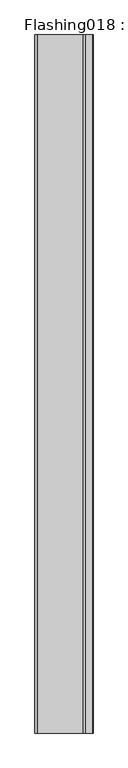
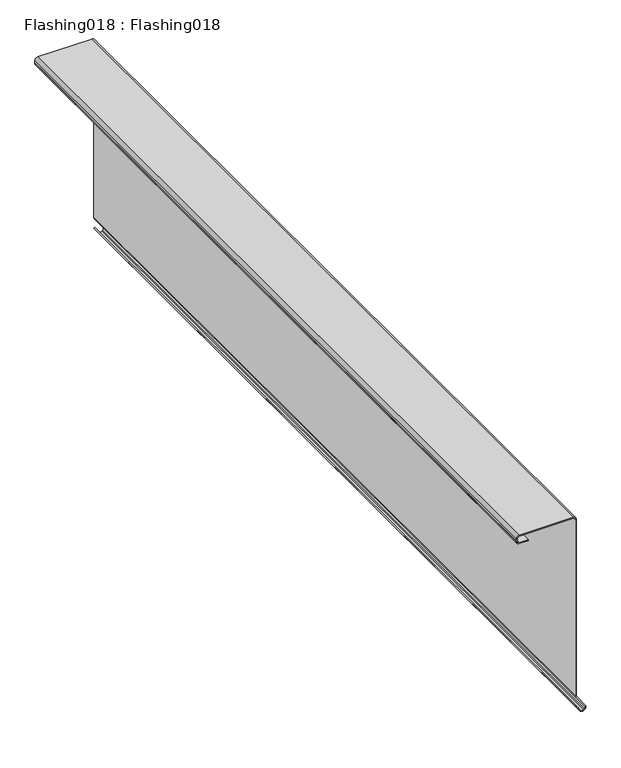
"""IFC4 building model written with IfcOpenShell, lengths in millimetres: proxy geometry, Flashing018 : Flashing018."""

from ifc_helpers import new_model, si_unit, point, frame, frame_2d, origin, place, context, project, spatial, polyline, circle_curve, trimmed, segment, composite_curve, outline, extrude, source, transform, mapped, element, save


def flashing018_flashing018_9543aaf0(model_context):
    return source(origin(), model_context, "Body", "SweptSolid", [
        extrude(outline(composite_curve([segment(polyline([(43036.8907248, 17759.2743151), (43051.477598, 17749.0170677), (43050.3271805, 17747.3810543), (43035.7403074, 17757.6383018)]), True, "CONTINUOUS"), segment(trimmed(circle_curve(frame_2d((43039.8127852, 17763.429789)), 7.08), [point((43035.7403074, 17757.6383018))], [point((43034.0825771, 17767.5880476))], False, "CARTESIAN"), True, "CONTINUOUS"), segment(polyline([(43034.0825771, 17767.5880476), (43035.3752562, 17769.3693991)]), True, "CONTINUOUS"), segment(trimmed(circle_curve(frame_2d((43041.1054643, 17765.2111405)), 7.08), [point((43035.3752562, 17769.3693991))], [point((43045.1570771, 17771.0172436))], False, "CARTESIAN"), True, "CONTINUOUS"), segment(polyline([(43045.1570771, 17771.0172436), (43075.4099277, 17749.9062098)]), True, "CONTINUOUS"), segment(trimmed(circle_curve(frame_2d((43077.1724938, 17752.4320286)), 3.08), [point((43075.4099277, 17749.9062098))], [point((43077.1724938, 17749.3520286))], True, "CARTESIAN"), True, "CONTINUOUS"), segment(polyline([(43077.1724938, 17749.3520286), (43524.4015043, 17749.3520286)]), True, "CONTINUOUS"), segment(trimmed(circle_curve(frame_2d((43524.4015043, 17742.2720286)), 7.08), [point((43524.4015043, 17749.3520286))], [point((43531.4815043, 17742.2720286))], False, "CARTESIAN"), True, "CONTINUOUS"), segment(polyline([(43531.4815043, 17742.2720286), (43531.4815043, 17612.9320286)]), True, "CONTINUOUS"), segment(trimmed(circle_curve(frame_2d((43524.4015043, 17612.9320286)), 7.08), [point((43531.4815043, 17612.9320286))], [point((43524.4015043, 17605.8520286))], False, "CARTESIAN"), True, "CONTINUOUS"), segment(polyline([(43524.4015043, 17605.8520286), (43517.995098, 17605.8520286)]), True, "CONTINUOUS"), segment(trimmed(circle_curve(frame_2d((43517.995098, 17612.9320286)), 7.08), [point((43517.995098, 17605.8520286))], [point((43510.915098, 17612.9320286))], False, "CARTESIAN"), True, "CONTINUOUS"), segment(polyline([(43510.915098, 17612.9320286), (43510.915098, 17634.2284935), (43512.915098, 17634.2284935), (43512.915098, 17612.9320286)]), True, "CONTINUOUS"), segment(trimmed(circle_curve(frame_2d((43517.995098, 17612.9320286)), 5.08), [point((43512.915098, 17612.9320286))], [point((43517.995098, 17607.8520286))], True, "CARTESIAN"), True, "CONTINUOUS"), segment(polyline([(43517.995098, 17607.8520286), (43524.4015043, 17607.8520286)]), True, "CONTINUOUS"), segment(trimmed(circle_curve(frame_2d((43524.4015043, 17612.9320286)), 5.08), [point((43524.4015043, 17607.8520286))], [point((43529.4815043, 17612.9320286))], True, "CARTESIAN"), True, "CONTINUOUS"), segment(polyline([(43529.4815043, 17612.9320286), (43529.4815043, 17742.2720286)]), True, "CONTINUOUS"), segment(trimmed(circle_curve(frame_2d((43524.4015043, 17742.2720286)), 5.08), [point((43529.4815043, 17742.2720286))], [point((43524.4015043, 17747.3520286))], True, "CARTESIAN"), True, "CONTINUOUS"), segment(polyline([(43524.4015043, 17747.3520286), (43077.1724938, 17747.3520286)]), True, "CONTINUOUS"), segment(trimmed(circle_curve(frame_2d((43077.1724938, 17752.4320286)), 5.08), [point((43077.1724938, 17747.3520286))], [point((43074.2654043, 17748.2660676))], False, "CARTESIAN"), True, "CONTINUOUS"), segment(polyline([(43074.2654043, 17748.2660676), (43044.0125537, 17769.3771014)]), True, "CONTINUOUS"), segment(trimmed(circle_curve(frame_2d((43041.1054643, 17765.2111405)), 5.08), [point((43044.0125537, 17769.3771014))], [point((43036.993959, 17768.1947498))], True, "CARTESIAN"), True, "CONTINUOUS"), segment(polyline([(43036.993959, 17768.1947498), (43035.7012799, 17766.4133983)]), True, "CONTINUOUS"), segment(trimmed(circle_curve(frame_2d((43039.8127852, 17763.429789)), 5.08), [point((43035.7012799, 17766.4133983))], [point((43036.8907248, 17759.2743151))], True, "CARTESIAN"), True, "CONTINUOUS")], self_intersect=False)), frame((0.0, 7982.1507711, 0.0), z_axis=(0.0, 1.0, 0.0), x_axis=(0.0, 0.0, 1.0)), (0.0, 0.0, 1.0), 2000.0),
    ])


if __name__ == "__main__":
    model = new_model("IFC4")
    model_context = context("Model", 3, world=origin())
    ifc_project = project(units=[si_unit("LENGTHUNIT", "METRE", prefix="MILLI")], contexts=[model_context])
    site = spatial("IfcSite", under=ifc_project)
    building = spatial("IfcBuilding", under=site)
    placement = place(None, origin())
    flashing018_flashing018_shape = flashing018_flashing018_9543aaf0(model_context)
    element("IfcBuildingElementProxy", 1, Name="Flashing018 : Flashing018", ObjectType="Flashing018 : Flashing018", at=placement, inside=building, context=model_context, shape_type="MappedRepresentation", body=[
        mapped(flashing018_flashing018_shape, transform((0.0, 0.0, 0.0), x_axis=(1.0, 0.0, 0.0), y_axis=(0.0, 1.0, 0.0), z_axis=(0.0, 0.0, 1.0))),
    ])
    save(model, "model.ifc")

# Revit data of these elements
# Type "Flashing018 : Flashing018"
#   NameOverride = "Flashing018"
# Element 1 (IfcBuildingElementProxy, "Flashing018 : Flashing018")
#   Materials on its faces: "HIGH EAVE FLASHING"
# Materials
#   "HIGH EAVE FLASHING": class "Unassigned", colour RGB 128 128 128, transparency 0, Cost = 0
